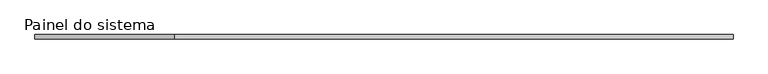
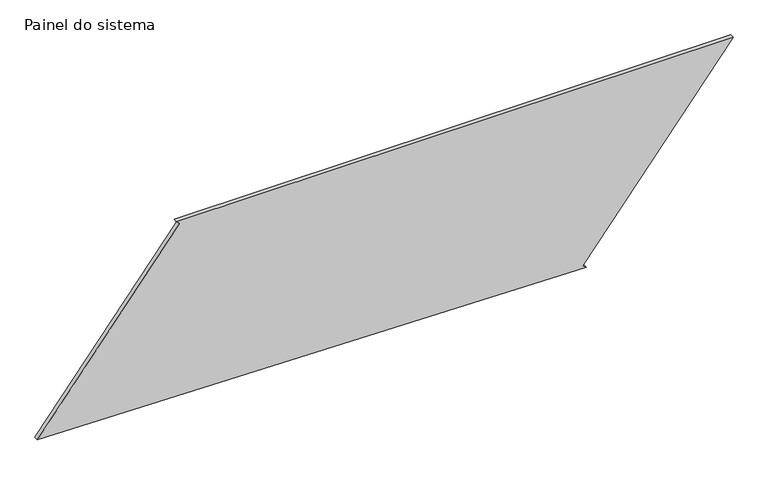
"""IFC4 building model written with IfcOpenShell, lengths in millimetres: plate geometry, Painel do sistema : Envidraçado."""

import ifcopenshell
import ifcopenshell.guid

model = None  # the IFC model being written
_history = None  # IfcOwnerHistory: only IFC2X3 demands one
_inside = {}  # id of a spatial element -> (the spatial element, [elements in it])
_under = {}  # id of a project, library or spatial element -> (it, [spatial elements below it])
_declared = {}  # id of a project -> (the project, [libraries it declares])
_typed = {}  # id of a type object -> (the type object, [elements of that type])
_made_of = {}  # id of a material, layer set ... -> (it, [elements and type objects made of it])


def new_model(schema):
    """Start an empty IFC model of exactly this schema.

    Asked for "IFC4X3", IfcOpenShell would pick the latest addendum, in which some entities
    have other attributes; the version numbers below select the first issue.
    IFC2X3 requires an IfcOwnerHistory on every rooted entity: one is made here for all.
    """
    global model, _history
    if schema == "IFC4X3":
        model = ifcopenshell.file(schema_version=(4, 3, 0, 0))
    else:
        model = ifcopenshell.file(schema=schema)
    _inside.clear()
    _under.clear()
    _declared.clear()
    _typed.clear()
    _made_of.clear()
    _history = None
    if model.schema == "IFC2X3":
        org = make("IfcOrganization", Name="unknown")
        user = make(
            "IfcPersonAndOrganization",
            ThePerson=make("IfcPerson", FamilyName="unknown"),
            TheOrganization=org,
        )
        app = make(
            "IfcApplication",
            ApplicationDeveloper=org,
            Version="unknown",
            ApplicationFullName="unknown",
            ApplicationIdentifier="unknown",
        )
        _history = make(
            "IfcOwnerHistory",
            OwningUser=user,
            OwningApplication=app,
            ChangeAction="ADDED",
            CreationDate=0,
        )
    return model


def make(cls, **values):
    """One entity of the class cls with the attributes given. An attribute that is None is left unset."""
    return model.create_entity(
        cls, **{name: value for name, value in values.items() if value is not None}
    )


def rooted(cls, **values):
    """An entity with a GlobalId (a new one), such as an element, a storey or a relation."""
    return make(cls, GlobalId=ifcopenshell.guid.new(), OwnerHistory=_history, **values)


def si_unit(unit_type, name, prefix=None):
    """IfcSIUnit, for example si_unit("LENGTHUNIT", "METRE", prefix="MILLI")."""
    return make("IfcSIUnit", UnitType=unit_type, Prefix=prefix, Name=name)


def assignment(units):
    """IfcUnitAssignment: the units of a project."""
    return None if units is None else make("IfcUnitAssignment", Units=units)


def point(xyz):
    """IfcCartesianPoint."""
    return None if xyz is None else make("IfcCartesianPoint", Coordinates=xyz)


def direction(xyz):
    """IfcDirection."""
    return None if xyz is None else make("IfcDirection", DirectionRatios=xyz)


def frame(location, z_axis=None, x_axis=None):
    """IfcAxis2Placement3D, a coordinate frame: its origin and axes. An axis left out is left unset."""
    return make(
        "IfcAxis2Placement3D",
        Location=point(location),
        Axis=direction(z_axis),
        RefDirection=direction(x_axis),
    )


def origin():
    """The frame at (0, 0, 0) with its axes left unset."""
    return frame((0.0, 0.0, 0.0))


def place(relative_to, where):
    """IfcLocalPlacement: puts the frame where relative to a parent placement (None: the world)."""
    return make(
        "IfcLocalPlacement", PlacementRelTo=relative_to, RelativePlacement=where
    )


def context(
    kind, dimensions, precision=None, world=None, true_north=None, identifier=None
):
    """IfcGeometricRepresentationContext, for example the 3D "Model" context."""
    return make(
        "IfcGeometricRepresentationContext",
        ContextIdentifier=identifier,
        ContextType=kind,
        CoordinateSpaceDimension=dimensions,
        Precision=precision,
        WorldCoordinateSystem=world,
        TrueNorth=true_north,
    )


def project(units=None, contexts=None):
    """IfcProject with its units and contexts."""
    return rooted(
        "IfcProject",
        Name="project",
        RepresentationContexts=contexts,
        UnitsInContext=assignment(units),
    )


def spatial(cls, under=None, at=None, **own):
    """A site, building, storey or space (cls), placed at a placement, below another one or the project."""
    s = rooted(cls, ObjectPlacement=at, **own)
    if under is not None:
        _under.setdefault(under.id(), (under, []))[1].append(s)
    return s


def polyline(points):
    """IfcPolyline through the points."""
    return make("IfcPolyline", Points=[point(p) for p in points])


def outline(outer, holes=None, kind="AREA"):
    """IfcArbitraryClosedProfileDef: a profile drawn as a closed curve; with holes, ...WithVoids."""
    if holes is None:
        return make("IfcArbitraryClosedProfileDef", ProfileType=kind, OuterCurve=outer)
    return make(
        "IfcArbitraryProfileDefWithVoids",
        ProfileType=kind,
        OuterCurve=outer,
        InnerCurves=holes,
    )


def extrude(swept, where, along, depth):
    """IfcExtrudedAreaSolid: the profile swept, set in the frame where, extruded along a direction by depth."""
    return make(
        "IfcExtrudedAreaSolid",
        SweptArea=swept,
        Position=where,
        ExtrudedDirection=direction(along),
        Depth=depth,
    )


def shape(context_of_items, identifier, shape_type, items):
    """IfcShapeRepresentation: the items that make up one representation, for example the "Body"."""
    return make(
        "IfcShapeRepresentation",
        ContextOfItems=context_of_items,
        RepresentationIdentifier=identifier,
        RepresentationType=shape_type,
        Items=items,
    )


def source(mapping_origin, context_of_items, identifier, shape_type, items):
    """IfcRepresentationMap: a shape defined once, which mapped items show again and again."""
    return make(
        "IfcRepresentationMap",
        MappingOrigin=mapping_origin,
        MappedRepresentation=shape(context_of_items, identifier, shape_type, items),
    )


def transform(
    local_origin,
    x_axis=None,
    y_axis=None,
    z_axis=None,
    scale=None,
    scale2=None,
    scale3=None,
    uniform=True,
):
    """IfcCartesianTransformationOperator3D, or its non-uniform kind. x_axis, y_axis, z_axis: its Axis1, 2, 3."""
    if uniform:
        return make(
            "IfcCartesianTransformationOperator3D",
            Axis1=direction(x_axis),
            Axis2=direction(y_axis),
            LocalOrigin=point(local_origin),
            Scale=scale,
            Axis3=direction(z_axis),
        )
    return make(
        "IfcCartesianTransformationOperator3DnonUniform",
        Axis1=direction(x_axis),
        Axis2=direction(y_axis),
        LocalOrigin=point(local_origin),
        Scale=scale,
        Axis3=direction(z_axis),
        Scale2=scale2,
        Scale3=scale3,
    )


def mapped(mapping_source, mapping_target):
    """IfcMappedItem: shows the shape of a source again, moved by a transform."""
    return make(
        "IfcMappedItem", MappingSource=mapping_source, MappingTarget=mapping_target
    )


def made_of(thing, what):
    """Note that an element or type object is made of a material, layer set ...; save() writes the relation."""
    if what is not None:
        _made_of.setdefault(what.id(), (what, []))[1].append(thing)
    return thing


def element(
    cls,
    number,
    at=None,
    inside=None,
    cuts=None,
    type_object=None,
    material=None,
    context=None,
    identifier="Body",
    shape_type=None,
    held_by="IfcProductDefinitionShape",
    body=None,
    shapes=None,
    **own,
):
    """One element of the class cls, such as IfcWall. Its Tag is "e" and its number.

    at: its placement. inside: the storey or other place that contains it. cuts: it is an
    opening in that element (IfcRelVoidsElement). A single representation is given by context,
    identifier, shape_type and body (its items); several are given by shapes. held_by: the class
    of the entity that holds the representations. save() writes the other relations.
    """
    e = rooted(cls, Tag="e%d" % number, ObjectPlacement=at, **own)
    if body is not None:
        shapes = [shape(context, identifier, shape_type, body)]
    if shapes is not None:
        e.Representation = make(held_by, Representations=shapes)
    if inside is not None:
        _inside.setdefault(inside.id(), (inside, []))[1].append(e)
    if cuts is not None:
        rooted(
            "IfcRelVoidsElement", RelatingBuildingElement=cuts, RelatedOpeningElement=e
        )
    if type_object is not None:
        _typed.setdefault(type_object.id(), (type_object, []))[1].append(e)
    return made_of(e, material)


def aggregate(whole, parts):
    """IfcRelAggregates: a whole, such as a stair, and the parts it consists of."""
    return rooted("IfcRelAggregates", RelatingObject=whole, RelatedObjects=parts)


def save(model, path):
    """Write the relations noted so far, then the file.

    IfcRelAggregates (storeys below a building ...), IfcRelContainedInSpatialStructure (elements
    in a storey), IfcRelDefinesByType, IfcRelAssociatesMaterial and IfcRelDeclares: one each for
    every whole, place, type object, material and project.
    """
    for whole, parts in _under.values():
        aggregate(whole, parts)
    for where, things in _inside.values():
        rooted(
            "IfcRelContainedInSpatialStructure",
            RelatedElements=things,
            RelatingStructure=where,
        )
    for kind, things in _typed.values():
        rooted("IfcRelDefinesByType", RelatedObjects=things, RelatingType=kind)
    for what, things in _made_of.values():
        rooted("IfcRelAssociatesMaterial", RelatedObjects=things, RelatingMaterial=what)
    for by, libraries in _declared.values():
        rooted("IfcRelDeclares", RelatingContext=by, RelatedDefinitions=libraries)
    model.write(path)


def painel_do_sistema_7230f658(model_context):
    return source(origin(), model_context, "Body", "SweptSolid", [
        extrude(outline(polyline([(0.0, 1174.9030197), (15.5601026, 1155.3356181), (1120.7892415, 2034.2197512), (1120.7892415, -1220.7205143), (1105.2291389, -1201.1531126), (57.6171855, -2034.2197512), (0.0, 1174.9030197)])), frame((0.0, 24.5, 0.0), z_axis=(0.0, 1.0, 0.0), x_axis=(0.0, 0.0, 1.0)), (0.0, 0.0, 1.0), 25.0),
    ])


if __name__ == "__main__":
    model = new_model("IFC4")
    model_context = context("Model", 3, world=origin())
    ifc_project = project(units=[si_unit("LENGTHUNIT", "METRE", prefix="MILLI")], contexts=[model_context])
    site = spatial("IfcSite", under=ifc_project)
    building = spatial("IfcBuilding", under=site)
    placement = place(None, origin())
    painel_do_sistema_shape = painel_do_sistema_7230f658(model_context)
    element("IfcPlate", 1, ObjectType="Painel do sistema : Envidraçado", at=placement, inside=building, context=model_context, shape_type="MappedRepresentation", body=[
        mapped(painel_do_sistema_shape, transform((0.0, 0.0, 0.0), x_axis=(1.0, 0.0, 0.0), y_axis=(0.0, 1.0, 0.0), z_axis=(0.0, 0.0, 1.0))),
    ])
    save(model, "model.ifc")

# Revit data of these elements
# Type "Painel do sistema : Envidraçado"
#   Construction Type Id = "GSP4R"
#   Analytic Construction = "Vidraça única Pilkington 1/8 pol"
#   Visual Light Transmittance = 0.9
#   Solar Heat Gain Coefficient = 0.86
#   Heat Transfer Coefficient (U) = 6.7069 W/(m²·K)
# Element 1 (IfcPlate, "Painel do sistema : Envidraçado")
#   Materials on its faces: "Vidro"
# Materials
#   "Vidro": class "Vidro", colour RGB 0 128 192, transparency 0.9, Description = "Vidro de sílica", Cost = 0
